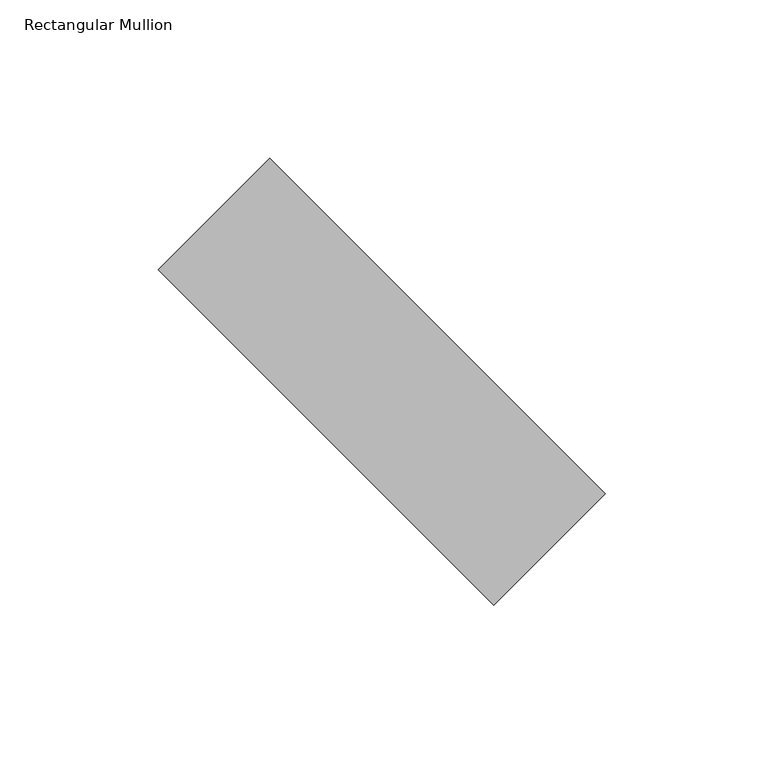
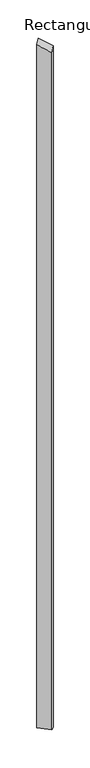
"""IFC4 building model written with IfcOpenShell, lengths in millimetres: member geometry, Rectangular Mullion : tilted mullions."""

import ifcopenshell
import ifcopenshell.guid

model = None  # the IFC model being written
_history = None  # IfcOwnerHistory: only IFC2X3 demands one
_inside = {}  # id of a spatial element -> (the spatial element, [elements in it])
_under = {}  # id of a project, library or spatial element -> (it, [spatial elements below it])
_declared = {}  # id of a project -> (the project, [libraries it declares])
_typed = {}  # id of a type object -> (the type object, [elements of that type])
_made_of = {}  # id of a material, layer set ... -> (it, [elements and type objects made of it])


def new_model(schema):
    """Start an empty IFC model of exactly this schema.

    Asked for "IFC4X3", IfcOpenShell would pick the latest addendum, in which some entities
    have other attributes; the version numbers below select the first issue.
    IFC2X3 requires an IfcOwnerHistory on every rooted entity: one is made here for all.
    """
    global model, _history
    if schema == "IFC4X3":
        model = ifcopenshell.file(schema_version=(4, 3, 0, 0))
    else:
        model = ifcopenshell.file(schema=schema)
    _inside.clear()
    _under.clear()
    _declared.clear()
    _typed.clear()
    _made_of.clear()
    _history = None
    if model.schema == "IFC2X3":
        org = make("IfcOrganization", Name="unknown")
        user = make(
            "IfcPersonAndOrganization",
            ThePerson=make("IfcPerson", FamilyName="unknown"),
            TheOrganization=org,
        )
        app = make(
            "IfcApplication",
            ApplicationDeveloper=org,
            Version="unknown",
            ApplicationFullName="unknown",
            ApplicationIdentifier="unknown",
        )
        _history = make(
            "IfcOwnerHistory",
            OwningUser=user,
            OwningApplication=app,
            ChangeAction="ADDED",
            CreationDate=0,
        )
    return model


def make(cls, **values):
    """One entity of the class cls with the attributes given. An attribute that is None is left unset."""
    return model.create_entity(
        cls, **{name: value for name, value in values.items() if value is not None}
    )


def rooted(cls, **values):
    """An entity with a GlobalId (a new one), such as an element, a storey or a relation."""
    return make(cls, GlobalId=ifcopenshell.guid.new(), OwnerHistory=_history, **values)


def si_unit(unit_type, name, prefix=None):
    """IfcSIUnit, for example si_unit("LENGTHUNIT", "METRE", prefix="MILLI")."""
    return make("IfcSIUnit", UnitType=unit_type, Prefix=prefix, Name=name)


def assignment(units):
    """IfcUnitAssignment: the units of a project."""
    return None if units is None else make("IfcUnitAssignment", Units=units)


def point(xyz):
    """IfcCartesianPoint."""
    return None if xyz is None else make("IfcCartesianPoint", Coordinates=xyz)


def direction(xyz):
    """IfcDirection."""
    return None if xyz is None else make("IfcDirection", DirectionRatios=xyz)


def frame(location, z_axis=None, x_axis=None):
    """IfcAxis2Placement3D, a coordinate frame: its origin and axes. An axis left out is left unset."""
    return make(
        "IfcAxis2Placement3D",
        Location=point(location),
        Axis=direction(z_axis),
        RefDirection=direction(x_axis),
    )


def origin():
    """The frame at (0, 0, 0) with its axes left unset."""
    return frame((0.0, 0.0, 0.0))


def place(relative_to, where):
    """IfcLocalPlacement: puts the frame where relative to a parent placement (None: the world)."""
    return make(
        "IfcLocalPlacement", PlacementRelTo=relative_to, RelativePlacement=where
    )


def context(
    kind, dimensions, precision=None, world=None, true_north=None, identifier=None
):
    """IfcGeometricRepresentationContext, for example the 3D "Model" context."""
    return make(
        "IfcGeometricRepresentationContext",
        ContextIdentifier=identifier,
        ContextType=kind,
        CoordinateSpaceDimension=dimensions,
        Precision=precision,
        WorldCoordinateSystem=world,
        TrueNorth=true_north,
    )


def project(units=None, contexts=None):
    """IfcProject with its units and contexts."""
    return rooted(
        "IfcProject",
        Name="project",
        RepresentationContexts=contexts,
        UnitsInContext=assignment(units),
    )


def spatial(cls, under=None, at=None, **own):
    """A site, building, storey or space (cls), placed at a placement, below another one or the project."""
    s = rooted(cls, ObjectPlacement=at, **own)
    if under is not None:
        _under.setdefault(under.id(), (under, []))[1].append(s)
    return s


def faces_of(points, faces, orient=None, outer=None):
    """IfcFace entities. A face is a list of loops; a loop is a list of indices into points, from 0.

    orient and outer hold one flag for each loop. By default every Orientation is true, the
    first loop of a face is its IfcFaceOuterBound and the others are IfcFaceBound.
    """
    made = []
    for i, loops in enumerate(faces):
        bounds = []
        for j, loop in enumerate(loops):
            is_outer = j == 0 if outer is None else outer[i][j]
            bounds.append(
                make(
                    "IfcFaceOuterBound" if is_outer else "IfcFaceBound",
                    Bound=make("IfcPolyLoop", Polygon=[points[k] for k in loop]),
                    Orientation=True if orient is None else orient[i][j],
                )
            )
        made.append(make("IfcFace", Bounds=bounds))
    return made


def faceted_brep(points, faces, orient=None, outer=None, voids=None):
    """IfcFacetedBrep: a solid bounded by flat faces; with voids (closed shells), ...WithVoids."""
    shared = [point(p) for p in points]
    hull = make("IfcClosedShell", CfsFaces=faces_of(shared, faces, orient, outer))
    if voids is None:
        return make("IfcFacetedBrep", Outer=hull)
    return make(
        "IfcFacetedBrepWithVoids",
        Outer=hull,
        Voids=[
            make(cls, CfsFaces=faces_of(shared, fs, o, b)) for cls, fs, o, b in voids
        ],
    )


def shape(context_of_items, identifier, shape_type, items):
    """IfcShapeRepresentation: the items that make up one representation, for example the "Body"."""
    return make(
        "IfcShapeRepresentation",
        ContextOfItems=context_of_items,
        RepresentationIdentifier=identifier,
        RepresentationType=shape_type,
        Items=items,
    )


def source(mapping_origin, context_of_items, identifier, shape_type, items):
    """IfcRepresentationMap: a shape defined once, which mapped items show again and again."""
    return make(
        "IfcRepresentationMap",
        MappingOrigin=mapping_origin,
        MappedRepresentation=shape(context_of_items, identifier, shape_type, items),
    )


def transform(
    local_origin,
    x_axis=None,
    y_axis=None,
    z_axis=None,
    scale=None,
    scale2=None,
    scale3=None,
    uniform=True,
):
    """IfcCartesianTransformationOperator3D, or its non-uniform kind. x_axis, y_axis, z_axis: its Axis1, 2, 3."""
    if uniform:
        return make(
            "IfcCartesianTransformationOperator3D",
            Axis1=direction(x_axis),
            Axis2=direction(y_axis),
            LocalOrigin=point(local_origin),
            Scale=scale,
            Axis3=direction(z_axis),
        )
    return make(
        "IfcCartesianTransformationOperator3DnonUniform",
        Axis1=direction(x_axis),
        Axis2=direction(y_axis),
        LocalOrigin=point(local_origin),
        Scale=scale,
        Axis3=direction(z_axis),
        Scale2=scale2,
        Scale3=scale3,
    )


def mapped(mapping_source, mapping_target):
    """IfcMappedItem: shows the shape of a source again, moved by a transform."""
    return make(
        "IfcMappedItem", MappingSource=mapping_source, MappingTarget=mapping_target
    )


def made_of(thing, what):
    """Note that an element or type object is made of a material, layer set ...; save() writes the relation."""
    if what is not None:
        _made_of.setdefault(what.id(), (what, []))[1].append(thing)
    return thing


def element(
    cls,
    number,
    at=None,
    inside=None,
    cuts=None,
    type_object=None,
    material=None,
    context=None,
    identifier="Body",
    shape_type=None,
    held_by="IfcProductDefinitionShape",
    body=None,
    shapes=None,
    **own,
):
    """One element of the class cls, such as IfcWall. Its Tag is "e" and its number.

    at: its placement. inside: the storey or other place that contains it. cuts: it is an
    opening in that element (IfcRelVoidsElement). A single representation is given by context,
    identifier, shape_type and body (its items); several are given by shapes. held_by: the class
    of the entity that holds the representations. save() writes the other relations.
    """
    e = rooted(cls, Tag="e%d" % number, ObjectPlacement=at, **own)
    if body is not None:
        shapes = [shape(context, identifier, shape_type, body)]
    if shapes is not None:
        e.Representation = make(held_by, Representations=shapes)
    if inside is not None:
        _inside.setdefault(inside.id(), (inside, []))[1].append(e)
    if cuts is not None:
        rooted(
            "IfcRelVoidsElement", RelatingBuildingElement=cuts, RelatedOpeningElement=e
        )
    if type_object is not None:
        _typed.setdefault(type_object.id(), (type_object, []))[1].append(e)
    return made_of(e, material)


def aggregate(whole, parts):
    """IfcRelAggregates: a whole, such as a stair, and the parts it consists of."""
    return rooted("IfcRelAggregates", RelatingObject=whole, RelatedObjects=parts)


def save(model, path):
    """Write the relations noted so far, then the file.

    IfcRelAggregates (storeys below a building ...), IfcRelContainedInSpatialStructure (elements
    in a storey), IfcRelDefinesByType, IfcRelAssociatesMaterial and IfcRelDeclares: one each for
    every whole, place, type object, material and project.
    """
    for whole, parts in _under.values():
        aggregate(whole, parts)
    for where, things in _inside.values():
        rooted(
            "IfcRelContainedInSpatialStructure",
            RelatedElements=things,
            RelatingStructure=where,
        )
    for kind, things in _typed.values():
        rooted("IfcRelDefinesByType", RelatedObjects=things, RelatingType=kind)
    for what, things in _made_of.values():
        rooted("IfcRelAssociatesMaterial", RelatedObjects=things, RelatingMaterial=what)
    for by, libraries in _declared.values():
        rooted("IfcRelDeclares", RelatingContext=by, RelatedDefinitions=libraries)
    model.write(path)


def rectangular_mullion_98a71f57(model_context):
    return source(origin(), model_context, "Body", "Brep", [
        faceted_brep([(-35.3553391, 70.7106781, -7999.3473161), (70.7106781, -35.3553391, -7999.3473161), (35.3553391, -70.7106781, -7999.3473161), (-70.7106781, 35.3553391, -7999.3473161), (-70.7106781, 35.3553391, 10.1224649), (-35.3553391, 70.7106781, 55.1417053), (35.3553391, -70.7106781, -55.1417053), (70.7106781, -35.3553391, -10.1224649)], [[[0, 1, 2, 3]], [[4, 5, 0, 3]], [[6, 4, 3, 2]], [[7, 6, 2, 1]], [[5, 7, 1, 0]], [[5, 4, 6, 7]]]),
    ])


if __name__ == "__main__":
    model = new_model("IFC4")
    model_context = context("Model", 3, world=origin())
    ifc_project = project(units=[si_unit("LENGTHUNIT", "METRE", prefix="MILLI")], contexts=[model_context])
    site = spatial("IfcSite", under=ifc_project)
    building = spatial("IfcBuilding", under=site)
    placement = place(None, origin())
    rectangular_mullion_shape = rectangular_mullion_98a71f57(model_context)
    element("IfcMember", 1, ObjectType="Rectangular Mullion : tilted mullions", at=placement, inside=building, context=model_context, shape_type="MappedRepresentation", body=[
        mapped(rectangular_mullion_shape, transform((0.0, 0.0, 0.0), x_axis=(1.0, 0.0, 0.0), y_axis=(0.0, 1.0, 0.0), z_axis=(0.0, 0.0, 1.0))),
    ])
    save(model, "model.ifc")

# Revit data of these elements
# Type "Rectangular Mullion : tilted mullions"
#   built-in parameter 1007304 = 0.492126 (stored number, unit not read)
#   built-in parameter 1007301 = 0.082021 (stored number, unit not read)
#   built-in parameter 1007300 = 0.082021 (stored number, unit not read)
# Element 1 (IfcMember, "Rectangular Mullion : tilted mullions")
#   Materials on its faces: "Aluminum"
# Materials
#   "Aluminum": class "Metal", colour RGB 244 244 244, transparency 0, Description = "Aluminum 6061", Cost = 0
